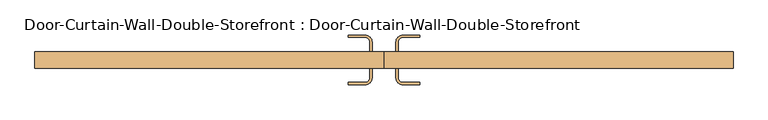
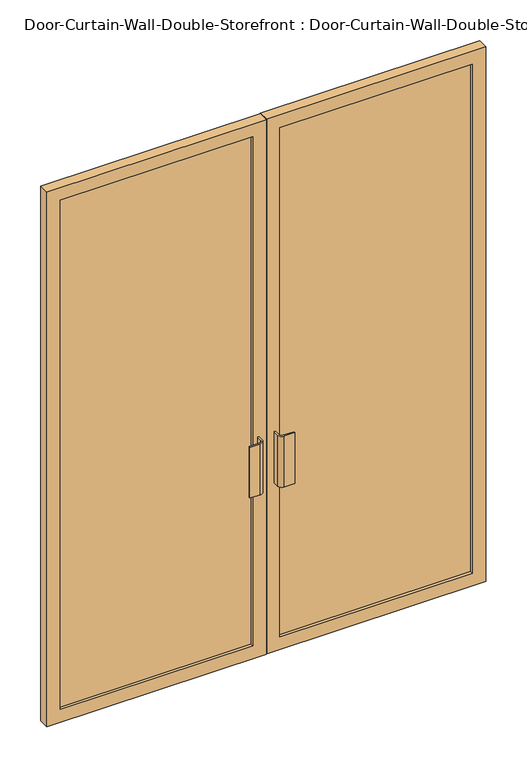
"""IFC4 building model written with IfcOpenShell, lengths in millimetres: door geometry, Door-Curtain-Wall-Double-Storefront : Door-Curtain-Wall-Double-Storefront."""

import ifcopenshell
import ifcopenshell.guid

model = None  # the IFC model being written
_history = None  # IfcOwnerHistory: only IFC2X3 demands one
_inside = {}  # id of a spatial element -> (the spatial element, [elements in it])
_under = {}  # id of a project, library or spatial element -> (it, [spatial elements below it])
_declared = {}  # id of a project -> (the project, [libraries it declares])
_typed = {}  # id of a type object -> (the type object, [elements of that type])
_made_of = {}  # id of a material, layer set ... -> (it, [elements and type objects made of it])


def new_model(schema):
    """Start an empty IFC model of exactly this schema.

    Asked for "IFC4X3", IfcOpenShell would pick the latest addendum, in which some entities
    have other attributes; the version numbers below select the first issue.
    IFC2X3 requires an IfcOwnerHistory on every rooted entity: one is made here for all.
    """
    global model, _history
    if schema == "IFC4X3":
        model = ifcopenshell.file(schema_version=(4, 3, 0, 0))
    else:
        model = ifcopenshell.file(schema=schema)
    _inside.clear()
    _under.clear()
    _declared.clear()
    _typed.clear()
    _made_of.clear()
    _history = None
    if model.schema == "IFC2X3":
        org = make("IfcOrganization", Name="unknown")
        user = make(
            "IfcPersonAndOrganization",
            ThePerson=make("IfcPerson", FamilyName="unknown"),
            TheOrganization=org,
        )
        app = make(
            "IfcApplication",
            ApplicationDeveloper=org,
            Version="unknown",
            ApplicationFullName="unknown",
            ApplicationIdentifier="unknown",
        )
        _history = make(
            "IfcOwnerHistory",
            OwningUser=user,
            OwningApplication=app,
            ChangeAction="ADDED",
            CreationDate=0,
        )
    return model


def make(cls, **values):
    """One entity of the class cls with the attributes given. An attribute that is None is left unset."""
    return model.create_entity(
        cls, **{name: value for name, value in values.items() if value is not None}
    )


def rooted(cls, **values):
    """An entity with a GlobalId (a new one), such as an element, a storey or a relation."""
    return make(cls, GlobalId=ifcopenshell.guid.new(), OwnerHistory=_history, **values)


def si_unit(unit_type, name, prefix=None):
    """IfcSIUnit, for example si_unit("LENGTHUNIT", "METRE", prefix="MILLI")."""
    return make("IfcSIUnit", UnitType=unit_type, Prefix=prefix, Name=name)


def assignment(units):
    """IfcUnitAssignment: the units of a project."""
    return None if units is None else make("IfcUnitAssignment", Units=units)


def point(xyz):
    """IfcCartesianPoint."""
    return None if xyz is None else make("IfcCartesianPoint", Coordinates=xyz)


def direction(xyz):
    """IfcDirection."""
    return None if xyz is None else make("IfcDirection", DirectionRatios=xyz)


def frame(location, z_axis=None, x_axis=None):
    """IfcAxis2Placement3D, a coordinate frame: its origin and axes. An axis left out is left unset."""
    return make(
        "IfcAxis2Placement3D",
        Location=point(location),
        Axis=direction(z_axis),
        RefDirection=direction(x_axis),
    )


def frame_2d(location, x_axis=None):
    """IfcAxis2Placement2D, a coordinate frame in the plane: its origin and x axis."""
    return make(
        "IfcAxis2Placement2D", Location=point(location), RefDirection=direction(x_axis)
    )


def origin():
    """The frame at (0, 0, 0) with its axes left unset."""
    return frame((0.0, 0.0, 0.0))


def place(relative_to, where):
    """IfcLocalPlacement: puts the frame where relative to a parent placement (None: the world)."""
    return make(
        "IfcLocalPlacement", PlacementRelTo=relative_to, RelativePlacement=where
    )


def context(
    kind, dimensions, precision=None, world=None, true_north=None, identifier=None
):
    """IfcGeometricRepresentationContext, for example the 3D "Model" context."""
    return make(
        "IfcGeometricRepresentationContext",
        ContextIdentifier=identifier,
        ContextType=kind,
        CoordinateSpaceDimension=dimensions,
        Precision=precision,
        WorldCoordinateSystem=world,
        TrueNorth=true_north,
    )


def project(units=None, contexts=None):
    """IfcProject with its units and contexts."""
    return rooted(
        "IfcProject",
        Name="project",
        RepresentationContexts=contexts,
        UnitsInContext=assignment(units),
    )


def spatial(cls, under=None, at=None, **own):
    """A site, building, storey or space (cls), placed at a placement, below another one or the project."""
    s = rooted(cls, ObjectPlacement=at, **own)
    if under is not None:
        _under.setdefault(under.id(), (under, []))[1].append(s)
    return s


def polyline(points):
    """IfcPolyline through the points."""
    return make("IfcPolyline", Points=[point(p) for p in points])


def circle_curve(where, radius):
    """IfcCircle in the frame where."""
    return make("IfcCircle", Position=where, Radius=radius)


def trimmed(basis, trim1, trim2, sense, master):
    """IfcTrimmedCurve: the piece of a basis curve between two trims."""
    return make(
        "IfcTrimmedCurve",
        BasisCurve=basis,
        Trim1=trim1,
        Trim2=trim2,
        SenseAgreement=sense,
        MasterRepresentation=master,
    )


def segment(curve, same_sense, transition):
    """IfcCompositeCurveSegment."""
    return make(
        "IfcCompositeCurveSegment",
        Transition=transition,
        SameSense=same_sense,
        ParentCurve=curve,
    )


def composite_curve(segments, self_intersect=None):
    """IfcCompositeCurve: segments joined end to end."""
    return make("IfcCompositeCurve", Segments=segments, SelfIntersect=self_intersect)


def outline(outer, holes=None, kind="AREA"):
    """IfcArbitraryClosedProfileDef: a profile drawn as a closed curve; with holes, ...WithVoids."""
    if holes is None:
        return make("IfcArbitraryClosedProfileDef", ProfileType=kind, OuterCurve=outer)
    return make(
        "IfcArbitraryProfileDefWithVoids",
        ProfileType=kind,
        OuterCurve=outer,
        InnerCurves=holes,
    )


def extrude(swept, where, along, depth):
    """IfcExtrudedAreaSolid: the profile swept, set in the frame where, extruded along a direction by depth."""
    return make(
        "IfcExtrudedAreaSolid",
        SweptArea=swept,
        Position=where,
        ExtrudedDirection=direction(along),
        Depth=depth,
    )


def shape(context_of_items, identifier, shape_type, items):
    """IfcShapeRepresentation: the items that make up one representation, for example the "Body"."""
    return make(
        "IfcShapeRepresentation",
        ContextOfItems=context_of_items,
        RepresentationIdentifier=identifier,
        RepresentationType=shape_type,
        Items=items,
    )


def source(mapping_origin, context_of_items, identifier, shape_type, items):
    """IfcRepresentationMap: a shape defined once, which mapped items show again and again."""
    return make(
        "IfcRepresentationMap",
        MappingOrigin=mapping_origin,
        MappedRepresentation=shape(context_of_items, identifier, shape_type, items),
    )


def transform(
    local_origin,
    x_axis=None,
    y_axis=None,
    z_axis=None,
    scale=None,
    scale2=None,
    scale3=None,
    uniform=True,
):
    """IfcCartesianTransformationOperator3D, or its non-uniform kind. x_axis, y_axis, z_axis: its Axis1, 2, 3."""
    if uniform:
        return make(
            "IfcCartesianTransformationOperator3D",
            Axis1=direction(x_axis),
            Axis2=direction(y_axis),
            LocalOrigin=point(local_origin),
            Scale=scale,
            Axis3=direction(z_axis),
        )
    return make(
        "IfcCartesianTransformationOperator3DnonUniform",
        Axis1=direction(x_axis),
        Axis2=direction(y_axis),
        LocalOrigin=point(local_origin),
        Scale=scale,
        Axis3=direction(z_axis),
        Scale2=scale2,
        Scale3=scale3,
    )


def mapped(mapping_source, mapping_target):
    """IfcMappedItem: shows the shape of a source again, moved by a transform."""
    return make(
        "IfcMappedItem", MappingSource=mapping_source, MappingTarget=mapping_target
    )


def made_of(thing, what):
    """Note that an element or type object is made of a material, layer set ...; save() writes the relation."""
    if what is not None:
        _made_of.setdefault(what.id(), (what, []))[1].append(thing)
    return thing


def element(
    cls,
    number,
    at=None,
    inside=None,
    cuts=None,
    type_object=None,
    material=None,
    context=None,
    identifier="Body",
    shape_type=None,
    held_by="IfcProductDefinitionShape",
    body=None,
    shapes=None,
    **own,
):
    """One element of the class cls, such as IfcWall. Its Tag is "e" and its number.

    at: its placement. inside: the storey or other place that contains it. cuts: it is an
    opening in that element (IfcRelVoidsElement). A single representation is given by context,
    identifier, shape_type and body (its items); several are given by shapes. held_by: the class
    of the entity that holds the representations. save() writes the other relations.
    """
    e = rooted(cls, Tag="e%d" % number, ObjectPlacement=at, **own)
    if body is not None:
        shapes = [shape(context, identifier, shape_type, body)]
    if shapes is not None:
        e.Representation = make(held_by, Representations=shapes)
    if inside is not None:
        _inside.setdefault(inside.id(), (inside, []))[1].append(e)
    if cuts is not None:
        rooted(
            "IfcRelVoidsElement", RelatingBuildingElement=cuts, RelatedOpeningElement=e
        )
    if type_object is not None:
        _typed.setdefault(type_object.id(), (type_object, []))[1].append(e)
    return made_of(e, material)


def aggregate(whole, parts):
    """IfcRelAggregates: a whole, such as a stair, and the parts it consists of."""
    return rooted("IfcRelAggregates", RelatingObject=whole, RelatedObjects=parts)


def save(model, path):
    """Write the relations noted so far, then the file.

    IfcRelAggregates (storeys below a building ...), IfcRelContainedInSpatialStructure (elements
    in a storey), IfcRelDefinesByType, IfcRelAssociatesMaterial and IfcRelDeclares: one each for
    every whole, place, type object, material and project.
    """
    for whole, parts in _under.values():
        aggregate(whole, parts)
    for where, things in _inside.values():
        rooted(
            "IfcRelContainedInSpatialStructure",
            RelatedElements=things,
            RelatingStructure=where,
        )
    for kind, things in _typed.values():
        rooted("IfcRelDefinesByType", RelatedObjects=things, RelatingType=kind)
    for what, things in _made_of.values():
        rooted("IfcRelAssociatesMaterial", RelatedObjects=things, RelatingMaterial=what)
    for by, libraries in _declared.values():
        rooted("IfcRelDeclares", RelatingContext=by, RelatedDefinitions=libraries)
    model.write(path)


def door_curtain_wall_double_storefront_door_curtain_wall_double_baac0ac5(model_context):
    return source(origin(), model_context, "Body", "SweptSolid", [
        extrude(outline(polyline([(2406.65, 0.7668501), (0.0, 0.7668501), (0.0, 933.45), (2406.65, 933.45), (2406.65, 0.7668501)]), holes=[polyline([(2349.5, 57.9168501), (2349.5, 876.3), (57.15, 876.3), (57.15, 57.9168501), (2349.5, 57.9168501)])]), frame((0.0, -57.15, 0.0), z_axis=(0.0, 1.0, 0.0), x_axis=(0.0, 0.0, 1.0)), (0.0, 0.0, 1.0), 44.45),
        extrude(outline(polyline([(2406.65, -0.8206499), (2406.65, -933.45), (0.0, -933.45), (0.0, -0.8206499), (2406.65, -0.8206499)]), holes=[polyline([(2349.5, -876.3), (2349.5, -57.9706499), (57.15, -57.9706499), (57.15, -876.3), (2349.5, -876.3)])]), frame((0.0, -57.15, 0.0), z_axis=(0.0, 1.0, 0.0), x_axis=(0.0, 0.0, 1.0)), (0.0, 0.0, 1.0), 44.45),
        extrude(outline(polyline([(876.3, -25.4), (876.3, -44.45), (57.9168501, -44.45), (57.9168501, -25.4), (876.3, -25.4)])), frame((0.0, 0.0, 57.15), z_axis=(0.0, 0.0, 1.0), x_axis=(1.0, 0.0, 0.0)), (0.0, 0.0, 1.0), 2292.35),
        extrude(outline(polyline([(-57.9706499, -25.4), (-57.9706499, -44.45), (-876.3, -44.45), (-876.3, -25.4), (-57.9706499, -25.4)])), frame((0.0, 0.0, 57.15), z_axis=(0.0, 0.0, 1.0), x_axis=(1.0, 0.0, 0.0)), (0.0, 0.0, 1.0), 2292.35),
        extrude(outline(composite_curve([segment(polyline([(-31.7768999, 12.7), (-31.7768999, -12.7), (-38.1268999, -12.7), (-38.1268999, 12.7)]), True, "CONTINUOUS"), segment(trimmed(circle_curve(frame_2d((-50.8268999, 12.7)), 12.7), [point((-38.1268999, 12.7))], [point((-50.8268999, 25.4))], True, "CARTESIAN"), True, "CONTINUOUS"), segment(polyline([(-50.8268999, 25.4), (-95.2768999, 25.4), (-95.2768999, 31.75), (-50.8268999, 31.75)]), True, "CONTINUOUS"), segment(trimmed(circle_curve(frame_2d((-50.8268999, 12.7)), 19.05), [point((-50.8268999, 31.75))], [point((-31.7768999, 12.7))], False, "CARTESIAN"), True, "CONTINUOUS")], self_intersect=False)), frame((0.0, 0.0, 762.0), z_axis=(0.0, 0.0, 1.0), x_axis=(1.0, 0.0, 0.0)), (0.0, 0.0, 1.0), 228.6),
        extrude(outline(composite_curve([segment(trimmed(circle_curve(frame_2d((50.7731001, 12.7)), 19.05), [point((31.7231001, 12.7))], [point((50.7731001, 31.75))], False, "CARTESIAN"), True, "CONTINUOUS"), segment(polyline([(50.7731001, 31.75), (95.2231001, 31.75), (95.2231001, 25.4), (50.7731001, 25.4)]), True, "CONTINUOUS"), segment(trimmed(circle_curve(frame_2d((50.7731001, 12.7)), 12.7), [point((50.7731001, 25.4))], [point((38.0731001, 12.7))], True, "CARTESIAN"), True, "CONTINUOUS"), segment(polyline([(38.0731001, 12.7), (38.0731001, -12.7), (31.7231001, -12.7), (31.7231001, 12.7)]), True, "CONTINUOUS")], self_intersect=False)), frame((0.0, 0.0, 762.0), z_axis=(0.0, 0.0, 1.0), x_axis=(1.0, 0.0, 0.0)), (0.0, 0.0, 1.0), 228.6),
        extrude(outline(composite_curve([segment(trimmed(circle_curve(frame_2d((-50.8268999, -82.55)), 19.05), [point((-31.7768999, -82.55))], [point((-50.8268999, -101.6))], False, "CARTESIAN"), True, "CONTINUOUS"), segment(polyline([(-50.8268999, -101.6), (-95.2768999, -101.6), (-95.2768999, -95.25), (-50.8268999, -95.25)]), True, "CONTINUOUS"), segment(trimmed(circle_curve(frame_2d((-50.8268999, -82.55)), 12.7), [point((-50.8268999, -95.25))], [point((-38.1268999, -82.55))], True, "CARTESIAN"), True, "CONTINUOUS"), segment(polyline([(-38.1268999, -82.55), (-38.1268999, -57.15), (-31.7768999, -57.15), (-31.7768999, -82.55)]), True, "CONTINUOUS")], self_intersect=False)), frame((0.0, 0.0, 762.0), z_axis=(0.0, 0.0, 1.0), x_axis=(1.0, 0.0, 0.0)), (0.0, 0.0, 1.0), 228.6),
        extrude(outline(composite_curve([segment(polyline([(31.7231001, -82.55), (31.7231001, -57.15), (38.0731001, -57.15), (38.0731001, -82.55)]), True, "CONTINUOUS"), segment(trimmed(circle_curve(frame_2d((50.7731001, -82.55)), 12.7), [point((38.0731001, -82.55))], [point((50.7731001, -95.25))], True, "CARTESIAN"), True, "CONTINUOUS"), segment(polyline([(50.7731001, -95.25), (95.2231001, -95.25), (95.2231001, -101.6), (50.7731001, -101.6)]), True, "CONTINUOUS"), segment(trimmed(circle_curve(frame_2d((50.7731001, -82.55)), 19.05), [point((50.7731001, -101.6))], [point((31.7231001, -82.55))], False, "CARTESIAN"), True, "CONTINUOUS")], self_intersect=False)), frame((0.0, 0.0, 762.0), z_axis=(0.0, 0.0, 1.0), x_axis=(1.0, 0.0, 0.0)), (0.0, 0.0, 1.0), 228.6),
    ])


if __name__ == "__main__":
    model = new_model("IFC4")
    model_context = context("Model", 3, world=origin())
    ifc_project = project(units=[si_unit("LENGTHUNIT", "METRE", prefix="MILLI")], contexts=[model_context])
    site = spatial("IfcSite", under=ifc_project)
    building = spatial("IfcBuilding", under=site)
    placement = place(None, origin())
    door_curtain_wall_double_storefront_door_curtain_wall_double_shape = door_curtain_wall_double_storefront_door_curtain_wall_double_baac0ac5(model_context)
    element("IfcDoor", 1, ObjectType="Door-Curtain-Wall-Double-Storefront : Door-Curtain-Wall-Double-Storefront", at=placement, inside=building, context=model_context, shape_type="MappedRepresentation", body=[
        mapped(door_curtain_wall_double_storefront_door_curtain_wall_double_shape, transform((0.0, 0.0, 0.0), x_axis=(1.0, 0.0, 0.0), y_axis=(0.0, 1.0, 0.0), z_axis=(0.0, 0.0, 1.0))),
    ])
    save(model, "model.ifc")

# Revit data of these elements
# Type "Door-Curtain-Wall-Double-Storefront : Door-Curtain-Wall-Double-Storefront"
#   Type Mark = "15"
#   Construction Type Id = "opn-d46"
#   Assembly Code = "B2030100"
#   Analytic Construction = "Metal frame, double glass door"
#   Width [instance default] = 6' - 0"
#   Thermal Resistance (R) = 1.3794 (h·ft²·°F)/BTU
#   Swing Angle [instance default] = 90.00°
#   Panel Width [instance default] = 3' - 0"
#   Offset = 0' - 2 1/4"
#   Heat Transfer Coefficient (U) = 0.7250 BTU/(h·ft²·°F)
#   Define Thermal Properties by = 1
#   Function = 1
#   Frame Material = Aluminum
#   Door Handle Material = Aluminum
#   Glazing = Glass
#   Visual Light Transmittance = 0
#   Solar Heat Gain Coefficient = 0
# Element 1 (IfcDoor, "Door-Curtain-Wall-Double-Storefront : Door-Curtain-Wall-Double-Storefront")
#   Width = 6' - 1 1/2"
#   Panel Width = 3' - 0 3/4"
#   Materials on its faces: "Aluminum", "Glass"
# Materials
#   "Aluminum": class "Metal", colour RGB 247 247 247, transparency 0, Description = "Aluminum 6061", Cost = 0
#   "Glass": class "Glass", colour RGB 0 0 255, transparency 0.75, Description = "Soda Lime Glass", Cost = 0
